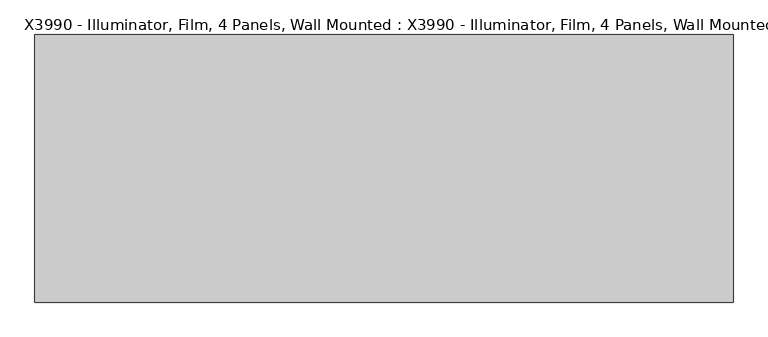
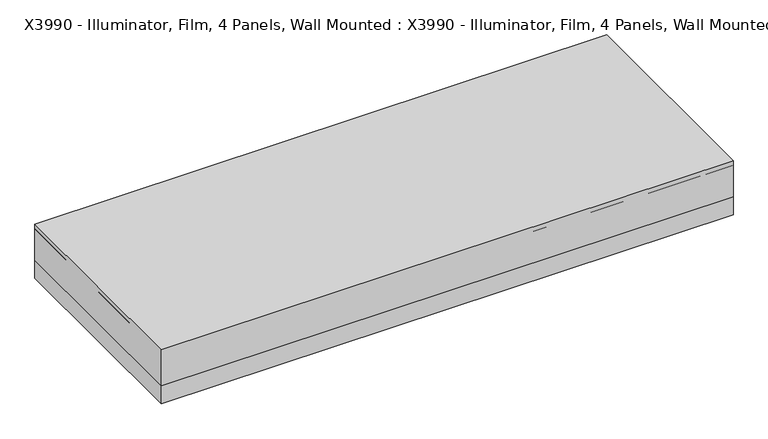
"""IFC4 building model written with IfcOpenShell, lengths in millimetres: proxy geometry, X3990 - Illuminator, Film, 4 Panels, Wall Mounted : X3990 - Illuminator, Film, 4 Panels, Wall Mounted."""

from ifc_helpers import new_model, si_unit, frame, origin, origin_with_axes, place, context, project, spatial, polyline, outline, extrude, source, transform, mapped, element, save


def x3990_illuminator_film_4_panels_wall_mounted_x3990_cb2436a7(model_context):
    return source(origin(), model_context, "Body", "SweptSolid", [
        extrude(outline(polyline([(-762.0, 292.1), (762.0, 292.1), (762.0, -292.1), (-762.0, -292.1), (-762.0, 292.1)])), frame((0.0, 0.0, 50.8), z_axis=(0.0, 0.0, 1.0), x_axis=(1.0, 0.0, 0.0)), (0.0, 0.0, 1.0), 101.6),
        extrude(outline(polyline([(660.4, 241.3), (660.4, 228.6), (-660.4, 228.6), (-660.4, 241.3), (660.4, 241.3)])), frame((0.0, 0.0, 139.7), z_axis=(0.0, 0.0, 1.0), x_axis=(1.0, 0.0, 0.0)), (0.0, 0.0, 1.0), 12.7),
        extrude(outline(polyline([(749.3, 228.6), (749.3, -273.7547399), (-749.3, -273.7547399), (-749.3, 228.6), (749.3, 228.6)])), origin_with_axes(), (0.0, 0.0, 1.0), 139.7),
        extrude(outline(polyline([(762.0, -292.1), (-762.0, -292.1), (-762.0, 292.1), (762.0, 292.1), (762.0, -292.1)]), holes=[polyline([(749.3, -273.7547399), (749.3, 228.6), (-749.3, 228.6), (-749.3, -273.7547399), (749.3, -273.7547399)])]), origin_with_axes(), (0.0, 0.0, 1.0), 139.7),
    ])


if __name__ == "__main__":
    model = new_model("IFC4")
    model_context = context("Model", 3, world=origin())
    ifc_project = project(units=[si_unit("LENGTHUNIT", "METRE", prefix="MILLI")], contexts=[model_context])
    site = spatial("IfcSite", under=ifc_project)
    building = spatial("IfcBuilding", under=site)
    placement = place(None, origin())
    x3990_illuminator_film_4_panels_wall_mounted_x3990_shape = x3990_illuminator_film_4_panels_wall_mounted_x3990_cb2436a7(model_context)
    element("IfcBuildingElementProxy", 1, Name="X3990 - Illuminator, Film, 4 Panels, Wall Mounted : X3990 - Illuminator, Film, 4 Panels, Wall Mounted", ObjectType="X3990 - Illuminator, Film, 4 Panels, Wall Mounted : X3990 - Illuminator, Film, 4 Panels, Wall Mounted", at=placement, inside=building, context=model_context, shape_type="MappedRepresentation", body=[
        mapped(x3990_illuminator_film_4_panels_wall_mounted_x3990_shape, transform((0.0, 0.0, 0.0), x_axis=(1.0, 0.0, 0.0), y_axis=(0.0, 1.0, 0.0), z_axis=(0.0, 0.0, 1.0))),
    ])
    save(model, "model.ifc")

# Revit data of these elements
# Type "X3990 - Illuminator, Film, 4 Panels, Wall Mounted : X3990 - Illuminator, Film, 4 Panels, Wall Mounted"
#   Watts2 = "0"
#   Watts1 = "600"
#   Unit_Issue = "EA"
#   UTIL_6_Misc = "-"
#   UTIL_5_NonMedGas = "-"
#   UTIL_4_MiscGas = "-"
#   UTIL_3_MedGas = "-"
#   UTIL_2_Elec = "A"
#   UTIL_1_WaterDrain = "-"
#   Nomenclature = "Illuminator, Film, 4 Panels, Wall Mounted"
#   NSN = "6525"
#   Location [instance default] = ""
#   JSN = "X3990"
#   Fund_Source_VA = "-"
#   Fund_Source_Navy = "-"
#   Fund_Source_Army = "-"
#   Fund_Source_AF = "-"
#   ELEC_Volts2 = "0"
#   ELEC_Volts1 = "120"
#   ELEC_Phase2 = "0"
#   ELEC_Phase1 = "1"
#   ELEC_HertzSwitch = "0"
#   ELEC_HertzDependent = "0"
#   ELEC_Hertz = "60"
#   ELEC_Amps2 = "0"
#   ELEC_Amps1 = "5"
#   DetailDescription = "Film illuminator, 4 panels, wall mounted. This unit is designed for simple on the wall installation. It has a front-mounted switch for independent control of fluorescent lamps. The unit is used to review and analyze radiography film in hospitals and X-ray clinics."
#   CAT_VA = "C"
#   CAT_Navy = "C"
#   CAT_IHS = "-"
#   CAT_Army = "C"
#   CAT_AF = "C"
#   BTUperhour = "0"
#   Weight_IP = 116
#   Default Elevation = 5' - 0"
#   DIM_Width_IP = 5' - 0"
#   DIM_Height_IP = 1' - 11"
#   DIM_Depth_IP = 0' - 6"
#   Assembly Code = ""
# Element 1 (IfcBuildingElementProxy, "X3990 - Illuminator, Film, 4 Panels, Wall Mounted : X3990 - Illuminator, Film, 4 Panels, Wall Mounted")
#   Materials on its faces: "EquipSpace", "Plastic - White"
# Materials
#   "EquipSpace": class "Unassigned", colour RGB 221 217 195, transparency 0.5
#   "Plastic - White": class "Unassigned", colour RGB 249 249 249, transparency 0
